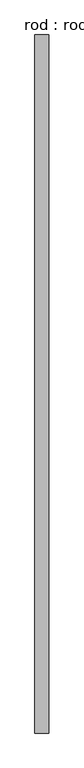
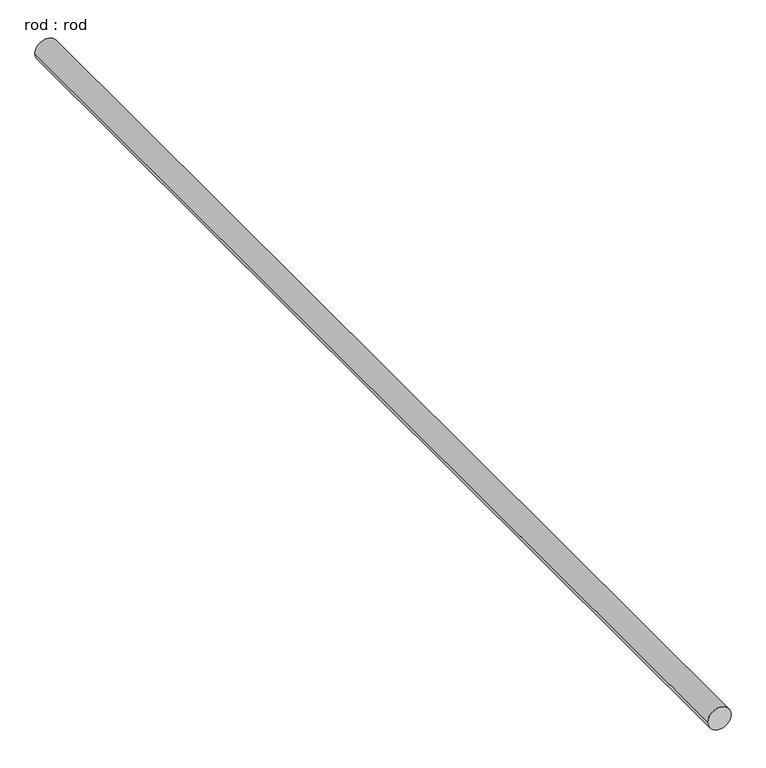
"""IFC4 building model written with IfcOpenShell, lengths in millimetres: proxy geometry, rod : rod."""

from ifc_helpers import new_model, si_unit, point, frame, frame_2d, origin, place, context, project, spatial, circle_curve, trimmed, segment, composite_curve, outline, extrude, source, transform, mapped, element, save


def rod_rod_bad7d949(model_context):
    return source(origin(), model_context, "Body", "SweptSolid", [
        extrude(outline(composite_curve([segment(trimmed(circle_curve(frame_2d((0.0108462, 0.0)), 200.0), [point((0.0108462, 200.0))], [point((0.0108462, -200.0))], False, "CARTESIAN"), True, "CONTINUOUS"), segment(trimmed(circle_curve(frame_2d((0.0108462, 0.0)), 200.0), [point((0.0108462, -200.0))], [point((0.0108462, 200.0))], False, "CARTESIAN"), True, "CONTINUOUS")], self_intersect=False)), frame((0.0, -5972.3719803, 0.0), z_axis=(0.0, 1.0, 0.0), x_axis=(0.0, 0.0, 1.0)), (0.0, 0.0, 1.0), 20130.2011912),
    ])


if __name__ == "__main__":
    model = new_model("IFC4")
    model_context = context("Model", 3, world=origin())
    ifc_project = project(units=[si_unit("LENGTHUNIT", "METRE", prefix="MILLI")], contexts=[model_context])
    site = spatial("IfcSite", under=ifc_project)
    building = spatial("IfcBuilding", under=site)
    placement = place(None, origin())
    rod_rod_shape = rod_rod_bad7d949(model_context)
    element("IfcBuildingElementProxy", 1, Name="rod : rod", ObjectType="rod : rod", at=placement, inside=building, context=model_context, shape_type="MappedRepresentation", body=[
        mapped(rod_rod_shape, transform((0.0, 0.0, 0.0), x_axis=(1.0, 0.0, 0.0), y_axis=(0.0, 1.0, 0.0), z_axis=(0.0, 0.0, 1.0))),
    ])
    save(model, "model.ifc")

# Revit data of these elements
# Type "rod : rod"
#   Default Elevation = 0
